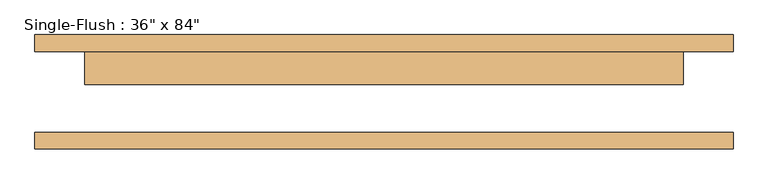
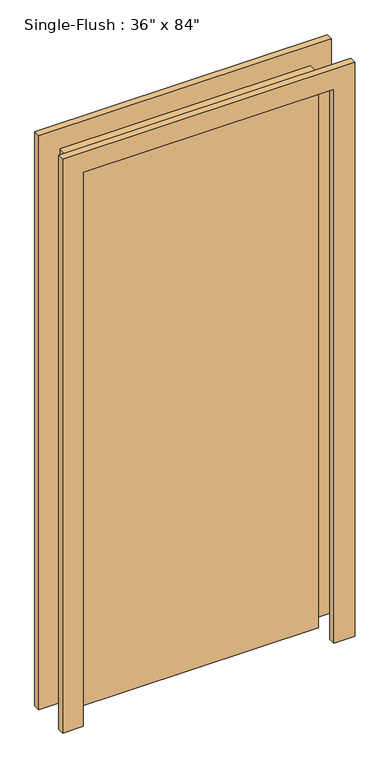
"""IFC4 building model written with IfcOpenShell, lengths in millimetres: door geometry."""

import ifcopenshell
import ifcopenshell.guid

model = None  # the IFC model being written
_history = None  # IfcOwnerHistory: only IFC2X3 demands one
_inside = {}  # id of a spatial element -> (the spatial element, [elements in it])
_under = {}  # id of a project, library or spatial element -> (it, [spatial elements below it])
_declared = {}  # id of a project -> (the project, [libraries it declares])
_typed = {}  # id of a type object -> (the type object, [elements of that type])
_made_of = {}  # id of a material, layer set ... -> (it, [elements and type objects made of it])


def new_model(schema):
    """Start an empty IFC model of exactly this schema.

    Asked for "IFC4X3", IfcOpenShell would pick the latest addendum, in which some entities
    have other attributes; the version numbers below select the first issue.
    IFC2X3 requires an IfcOwnerHistory on every rooted entity: one is made here for all.
    """
    global model, _history
    if schema == "IFC4X3":
        model = ifcopenshell.file(schema_version=(4, 3, 0, 0))
    else:
        model = ifcopenshell.file(schema=schema)
    _inside.clear()
    _under.clear()
    _declared.clear()
    _typed.clear()
    _made_of.clear()
    _history = None
    if model.schema == "IFC2X3":
        org = make("IfcOrganization", Name="unknown")
        user = make(
            "IfcPersonAndOrganization",
            ThePerson=make("IfcPerson", FamilyName="unknown"),
            TheOrganization=org,
        )
        app = make(
            "IfcApplication",
            ApplicationDeveloper=org,
            Version="unknown",
            ApplicationFullName="unknown",
            ApplicationIdentifier="unknown",
        )
        _history = make(
            "IfcOwnerHistory",
            OwningUser=user,
            OwningApplication=app,
            ChangeAction="ADDED",
            CreationDate=0,
        )
    return model


def make(cls, **values):
    """One entity of the class cls with the attributes given. An attribute that is None is left unset."""
    return model.create_entity(
        cls, **{name: value for name, value in values.items() if value is not None}
    )


def rooted(cls, **values):
    """An entity with a GlobalId (a new one), such as an element, a storey or a relation."""
    return make(cls, GlobalId=ifcopenshell.guid.new(), OwnerHistory=_history, **values)


def si_unit(unit_type, name, prefix=None):
    """IfcSIUnit, for example si_unit("LENGTHUNIT", "METRE", prefix="MILLI")."""
    return make("IfcSIUnit", UnitType=unit_type, Prefix=prefix, Name=name)


def assignment(units):
    """IfcUnitAssignment: the units of a project."""
    return None if units is None else make("IfcUnitAssignment", Units=units)


def point(xyz):
    """IfcCartesianPoint."""
    return None if xyz is None else make("IfcCartesianPoint", Coordinates=xyz)


def direction(xyz):
    """IfcDirection."""
    return None if xyz is None else make("IfcDirection", DirectionRatios=xyz)


def frame(location, z_axis=None, x_axis=None):
    """IfcAxis2Placement3D, a coordinate frame: its origin and axes. An axis left out is left unset."""
    return make(
        "IfcAxis2Placement3D",
        Location=point(location),
        Axis=direction(z_axis),
        RefDirection=direction(x_axis),
    )


def origin():
    """The frame at (0, 0, 0) with its axes left unset."""
    return frame((0.0, 0.0, 0.0))


def origin_with_axes():
    """The frame at (0, 0, 0) with the z axis (0, 0, 1) and the x axis (1, 0, 0) written out."""
    return frame((0.0, 0.0, 0.0), z_axis=(0.0, 0.0, 1.0), x_axis=(1.0, 0.0, 0.0))


def place(relative_to, where):
    """IfcLocalPlacement: puts the frame where relative to a parent placement (None: the world)."""
    return make(
        "IfcLocalPlacement", PlacementRelTo=relative_to, RelativePlacement=where
    )


def context(
    kind, dimensions, precision=None, world=None, true_north=None, identifier=None
):
    """IfcGeometricRepresentationContext, for example the 3D "Model" context."""
    return make(
        "IfcGeometricRepresentationContext",
        ContextIdentifier=identifier,
        ContextType=kind,
        CoordinateSpaceDimension=dimensions,
        Precision=precision,
        WorldCoordinateSystem=world,
        TrueNorth=true_north,
    )


def project(units=None, contexts=None):
    """IfcProject with its units and contexts."""
    return rooted(
        "IfcProject",
        Name="project",
        RepresentationContexts=contexts,
        UnitsInContext=assignment(units),
    )


def spatial(cls, under=None, at=None, **own):
    """A site, building, storey or space (cls), placed at a placement, below another one or the project."""
    s = rooted(cls, ObjectPlacement=at, **own)
    if under is not None:
        _under.setdefault(under.id(), (under, []))[1].append(s)
    return s


def polyline(points):
    """IfcPolyline through the points."""
    return make("IfcPolyline", Points=[point(p) for p in points])


def outline(outer, holes=None, kind="AREA"):
    """IfcArbitraryClosedProfileDef: a profile drawn as a closed curve; with holes, ...WithVoids."""
    if holes is None:
        return make("IfcArbitraryClosedProfileDef", ProfileType=kind, OuterCurve=outer)
    return make(
        "IfcArbitraryProfileDefWithVoids",
        ProfileType=kind,
        OuterCurve=outer,
        InnerCurves=holes,
    )


def extrude(swept, where, along, depth):
    """IfcExtrudedAreaSolid: the profile swept, set in the frame where, extruded along a direction by depth."""
    return make(
        "IfcExtrudedAreaSolid",
        SweptArea=swept,
        Position=where,
        ExtrudedDirection=direction(along),
        Depth=depth,
    )


def shape(context_of_items, identifier, shape_type, items):
    """IfcShapeRepresentation: the items that make up one representation, for example the "Body"."""
    return make(
        "IfcShapeRepresentation",
        ContextOfItems=context_of_items,
        RepresentationIdentifier=identifier,
        RepresentationType=shape_type,
        Items=items,
    )


def source(mapping_origin, context_of_items, identifier, shape_type, items):
    """IfcRepresentationMap: a shape defined once, which mapped items show again and again."""
    return make(
        "IfcRepresentationMap",
        MappingOrigin=mapping_origin,
        MappedRepresentation=shape(context_of_items, identifier, shape_type, items),
    )


def transform(
    local_origin,
    x_axis=None,
    y_axis=None,
    z_axis=None,
    scale=None,
    scale2=None,
    scale3=None,
    uniform=True,
):
    """IfcCartesianTransformationOperator3D, or its non-uniform kind. x_axis, y_axis, z_axis: its Axis1, 2, 3."""
    if uniform:
        return make(
            "IfcCartesianTransformationOperator3D",
            Axis1=direction(x_axis),
            Axis2=direction(y_axis),
            LocalOrigin=point(local_origin),
            Scale=scale,
            Axis3=direction(z_axis),
        )
    return make(
        "IfcCartesianTransformationOperator3DnonUniform",
        Axis1=direction(x_axis),
        Axis2=direction(y_axis),
        LocalOrigin=point(local_origin),
        Scale=scale,
        Axis3=direction(z_axis),
        Scale2=scale2,
        Scale3=scale3,
    )


def mapped(mapping_source, mapping_target):
    """IfcMappedItem: shows the shape of a source again, moved by a transform."""
    return make(
        "IfcMappedItem", MappingSource=mapping_source, MappingTarget=mapping_target
    )


def made_of(thing, what):
    """Note that an element or type object is made of a material, layer set ...; save() writes the relation."""
    if what is not None:
        _made_of.setdefault(what.id(), (what, []))[1].append(thing)
    return thing


def element(
    cls,
    number,
    at=None,
    inside=None,
    cuts=None,
    type_object=None,
    material=None,
    context=None,
    identifier="Body",
    shape_type=None,
    held_by="IfcProductDefinitionShape",
    body=None,
    shapes=None,
    **own,
):
    """One element of the class cls, such as IfcWall. Its Tag is "e" and its number.

    at: its placement. inside: the storey or other place that contains it. cuts: it is an
    opening in that element (IfcRelVoidsElement). A single representation is given by context,
    identifier, shape_type and body (its items); several are given by shapes. held_by: the class
    of the entity that holds the representations. save() writes the other relations.
    """
    e = rooted(cls, Tag="e%d" % number, ObjectPlacement=at, **own)
    if body is not None:
        shapes = [shape(context, identifier, shape_type, body)]
    if shapes is not None:
        e.Representation = make(held_by, Representations=shapes)
    if inside is not None:
        _inside.setdefault(inside.id(), (inside, []))[1].append(e)
    if cuts is not None:
        rooted(
            "IfcRelVoidsElement", RelatingBuildingElement=cuts, RelatedOpeningElement=e
        )
    if type_object is not None:
        _typed.setdefault(type_object.id(), (type_object, []))[1].append(e)
    return made_of(e, material)


def aggregate(whole, parts):
    """IfcRelAggregates: a whole, such as a stair, and the parts it consists of."""
    return rooted("IfcRelAggregates", RelatingObject=whole, RelatedObjects=parts)


def save(model, path):
    """Write the relations noted so far, then the file.

    IfcRelAggregates (storeys below a building ...), IfcRelContainedInSpatialStructure (elements
    in a storey), IfcRelDefinesByType, IfcRelAssociatesMaterial and IfcRelDeclares: one each for
    every whole, place, type object, material and project.
    """
    for whole, parts in _under.values():
        aggregate(whole, parts)
    for where, things in _inside.values():
        rooted(
            "IfcRelContainedInSpatialStructure",
            RelatedElements=things,
            RelatingStructure=where,
        )
    for kind, things in _typed.values():
        rooted("IfcRelDefinesByType", RelatedObjects=things, RelatingType=kind)
    for what, things in _made_of.values():
        rooted("IfcRelAssociatesMaterial", RelatedObjects=things, RelatingMaterial=what)
    for by, libraries in _declared.values():
        rooted("IfcRelDeclares", RelatingContext=by, RelatedDefinitions=libraries)
    model.write(path)


def door_88503111(model_context):
    return source(origin(), model_context, "Body", "SweptSolid", [
        extrude(outline(polyline([(2209.8, -533.4), (0.0, -533.4), (0.0, -457.2), (2133.6, -457.2), (2133.6, 457.2), (0.0, 457.2), (0.0, 533.4), (2209.8, 533.4), (2209.8, -533.4)])), frame((0.0, 61.9125, 0.0), z_axis=(0.0, 1.0, 0.0), x_axis=(0.0, 0.0, 1.0)), (0.0, 0.0, 1.0), 25.4),
        extrude(outline(polyline([(2209.8, 533.4), (2209.8, -533.4), (0.0, -533.4), (0.0, -457.2), (2133.6, -457.2), (2133.6, 457.2), (0.0, 457.2), (0.0, 533.4), (2209.8, 533.4)])), frame((0.0, -87.3125, 0.0), z_axis=(0.0, 1.0, 0.0), x_axis=(0.0, 0.0, 1.0)), (0.0, 0.0, 1.0), 25.4),
        extrude(outline(polyline([(457.2, 11.1125), (-457.2, 11.1125), (-457.2, 61.9125), (457.2, 61.9125), (457.2, 11.1125)])), origin_with_axes(), (0.0, 0.0, 1.0), 2133.6),
    ])


if __name__ == "__main__":
    model = new_model("IFC4")
    model_context = context("Model", 3, world=origin())
    ifc_project = project(units=[si_unit("LENGTHUNIT", "METRE", prefix="MILLI")], contexts=[model_context])
    site = spatial("IfcSite", under=ifc_project)
    building = spatial("IfcBuilding", under=site)
    placement = place(None, origin())
    door_shape = door_88503111(model_context)
    element("IfcDoor", 1, ObjectType="Single-Flush : 36\" x 84\"", at=placement, inside=building, context=model_context, shape_type="MappedRepresentation", body=[
        mapped(door_shape, transform((0.0, 0.0, 0.0), x_axis=(1.0, 0.0, 0.0), y_axis=(0.0, 1.0, 0.0), z_axis=(0.0, 0.0, 1.0))),
    ])
    save(model, "model.ifc")

# Revit data of these elements
# Type "Single-Flush : 36\" x 84\""
#   Type Mark = "1"
#   Construction Type = "A"
#   Construction Type = "A"
#   Assembly Code = "C1020"
#   Thickness = 0' - 2"
#   Height = 7' - 0"
#   Trim Projection Ext = 0' - 1"
#   Trim Projection Int = 0' - 1"
#   Trim Width = 0' - 3"
#   Width = 3' - 0"
#   Door Material = Door - Panel
#   Frame Material = Door - Frame
#   Function = (empty or 0)
#   Wall Closure = (empty or 0)
# Element 1 (IfcDoor, "Single-Flush : 36\" x 84\"")
#   Materials on its faces: "Door - Frame", "Door - Panel"
# Materials
#   "Door - Panel": class "Wood", colour RGB 210 159 95, transparency 0
#   "Door - Frame": class "Miscellaneous", colour RGB 118 70 51, transparency 0
